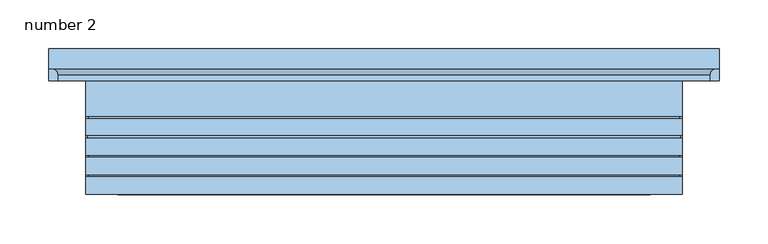
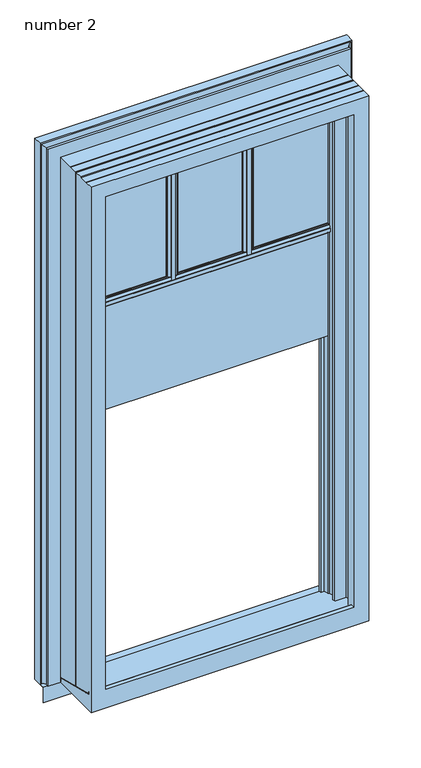
"""IFC4 building model written with IfcOpenShell, lengths in millimetres: window geometry, Window-Exterior-Sierra-Double_Hung-Operating_Unit-18inch_48inch-Width-(Hi-Divide) : number 2."""

from ifc_helpers import new_model, si_unit, point, frame, frame_2d, origin, place, context, project, spatial, polyline, circle_curve, ellipse_curve, trimmed, segment, composite_curve, outline, extrude, source, transform, mapped, element, save
from ifc_brep_helpers import plane_surface, cylinder_surface, revolved_surface, advanced_brep


def number_2_2d71ef64(model_context):
    return source(origin(), model_context, "Body", "SolidModel", [
        extrude(outline(composite_curve([segment(polyline([(-94.1939779, 37.8983982), (-94.1939779, 40.5653982), (-92.6191779, 40.5653982)]), True, "CONTINUOUS"), segment(trimmed(circle_curve(frame_2d((-87.3857184, 38.4281587)), 5.6530426), [point((-92.6191779, 40.5653982))], [point((-87.0396445, 44.0705982))], False, "CARTESIAN"), True, "CONTINUOUS"), segment(polyline([(-87.0396445, 44.0705982), (-87.0396445, 46.6296482), (-79.1233112, 46.6296482), (-79.1233112, 44.0705982)]), True, "CONTINUOUS"), segment(trimmed(circle_curve(frame_2d((-78.7772374, 38.4281587)), 5.6530426), [point((-79.1233112, 44.0705982))], [point((-73.5437779, 40.5653982))], False, "CARTESIAN"), True, "CONTINUOUS"), segment(polyline([(-73.5437779, 40.5653982), (-71.9689779, 40.5653982), (-71.9689779, 37.8983982), (-94.1939779, 37.8983982)]), True, "CONTINUOUS")], self_intersect=False)), frame((0.0, 0.0, 1795.5188733), z_axis=(0.0, 0.0, 1.0), x_axis=(1.0, 0.0, 0.0)), (0.0, 0.0, 1.0), 304.8),
        extrude(outline(composite_curve([segment(polyline([(-94.1939779, 18.8483982), (-71.9689779, 18.8483982), (-71.9689779, 16.1813982), (-73.5437779, 16.1813982)]), True, "CONTINUOUS"), segment(trimmed(circle_curve(frame_2d((-78.7772374, 18.3186378)), 5.6530426), [point((-73.5437779, 16.1813982))], [point((-79.1233112, 12.6761982))], False, "CARTESIAN"), True, "CONTINUOUS"), segment(polyline([(-79.1233112, 12.6761982), (-79.1233112, 10.1171482), (-87.0396445, 10.1171482), (-87.0396445, 12.6761982)]), True, "CONTINUOUS"), segment(trimmed(circle_curve(frame_2d((-87.3857184, 18.3186378)), 5.6530426), [point((-87.0396445, 12.6761982))], [point((-92.6191779, 16.1813982))], False, "CARTESIAN"), True, "CONTINUOUS"), segment(polyline([(-92.6191779, 16.1813982), (-94.1939779, 16.1813982), (-94.1939779, 18.8483982)]), True, "CONTINUOUS")], self_intersect=False)), frame((0.0, 0.0, 1795.5188733), z_axis=(0.0, 0.0, 1.0), x_axis=(1.0, 0.0, 0.0)), (0.0, 0.0, 1.0), 304.8),
        extrude(outline(composite_curve([segment(polyline([(-83.0927539, 18.8483982), (-71.9689779, 18.8483982), (-71.9689779, 14.5562974), (-73.5437779, 14.5562974)]), True, "CONTINUOUS"), segment(trimmed(circle_curve(frame_2d((-78.7772374, 18.3186378)), 6.445487), [point((-73.5437779, 14.5562974))], [point((-79.1233112, 11.8824482))], False, "CARTESIAN"), True, "CONTINUOUS"), segment(polyline([(-79.1233112, 11.8824482), (-79.1233112, 10.1171482), (-87.0396445, 10.1171482), (-87.0396445, 12.6761982)]), True, "CONTINUOUS"), segment(trimmed(circle_curve(frame_2d((-87.3857184, 18.3186378)), 5.6530426), [point((-87.0396445, 12.6761982))], [point((-92.6191779, 16.1813982))], False, "CARTESIAN"), True, "CONTINUOUS"), segment(polyline([(-92.6191779, 16.1813982), (-94.1939779, 16.1813982), (-94.1939779, 18.8483982), (-83.0927539, 18.8483982)]), True, "CONTINUOUS")], self_intersect=False)), frame((0.0, 0.0, 1795.5188733), z_axis=(0.0, 0.0, 1.0), x_axis=(1.0, 0.0, 0.0)), (0.0, 0.0, 1.0), 304.8),
        extrude(outline(composite_curve([segment(polyline([(71.9689779, 37.8983982), (71.9689779, 40.5653982), (73.5437779, 40.5653982)]), True, "CONTINUOUS"), segment(trimmed(circle_curve(frame_2d((78.7772374, 38.4281587)), 5.6530426), [point((73.5437779, 40.5653982))], [point((79.1233112, 44.0705982))], False, "CARTESIAN"), True, "CONTINUOUS"), segment(polyline([(79.1233112, 44.0705982), (79.1233112, 46.6296482), (87.0396445, 46.6296482), (87.0396445, 44.0705982)]), True, "CONTINUOUS"), segment(trimmed(circle_curve(frame_2d((87.3857184, 38.4281587)), 5.6530426), [point((87.0396445, 44.0705982))], [point((92.6191779, 40.5653982))], False, "CARTESIAN"), True, "CONTINUOUS"), segment(polyline([(92.6191779, 40.5653982), (94.1939779, 40.5653982), (94.1939779, 37.8983982), (71.9689779, 37.8983982)]), True, "CONTINUOUS")], self_intersect=False)), frame((0.0, 0.0, 1795.5188733), z_axis=(0.0, 0.0, 1.0), x_axis=(1.0, 0.0, 0.0)), (0.0, 0.0, 1.0), 304.8),
        extrude(outline(composite_curve([segment(polyline([(71.9689779, 18.8483982), (94.1939779, 18.8483982), (94.1939779, 16.1813982), (92.6191779, 16.1813982)]), True, "CONTINUOUS"), segment(trimmed(circle_curve(frame_2d((87.3857184, 18.3186378)), 5.6530426), [point((92.6191779, 16.1813982))], [point((87.0396445, 12.6761982))], False, "CARTESIAN"), True, "CONTINUOUS"), segment(polyline([(87.0396445, 12.6761982), (87.0396445, 10.1171482), (79.1233112, 10.1171482), (79.1233112, 12.6761982)]), True, "CONTINUOUS"), segment(trimmed(circle_curve(frame_2d((78.7772374, 18.3186378)), 5.6530426), [point((79.1233112, 12.6761982))], [point((73.5437779, 16.1813982))], False, "CARTESIAN"), True, "CONTINUOUS"), segment(polyline([(73.5437779, 16.1813982), (71.9689779, 16.1813982), (71.9689779, 18.8483982)]), True, "CONTINUOUS")], self_intersect=False)), frame((0.0, 0.0, 1795.5188733), z_axis=(0.0, 0.0, 1.0), x_axis=(1.0, 0.0, 0.0)), (0.0, 0.0, 1.0), 304.8),
        extrude(outline(composite_curve([segment(polyline([(83.0702018, 18.8483982), (94.1939779, 18.8483982), (94.1939779, 14.5562974), (92.6191779, 14.5562974)]), True, "CONTINUOUS"), segment(trimmed(circle_curve(frame_2d((87.3857184, 18.3186378)), 6.445487), [point((92.6191779, 14.5562974))], [point((87.0396445, 11.8824482))], False, "CARTESIAN"), True, "CONTINUOUS"), segment(polyline([(87.0396445, 11.8824482), (87.0396445, 10.1171482), (79.1233112, 10.1171482), (79.1233112, 12.6761982)]), True, "CONTINUOUS"), segment(trimmed(circle_curve(frame_2d((78.7772374, 18.3186378)), 5.6530426), [point((79.1233112, 12.6761982))], [point((73.5437779, 16.1813982))], False, "CARTESIAN"), True, "CONTINUOUS"), segment(polyline([(73.5437779, 16.1813982), (71.9689779, 16.1813982), (71.9689779, 18.8483982), (83.0702018, 18.8483982)]), True, "CONTINUOUS")], self_intersect=False)), frame((0.0, 0.0, 1795.5188733), z_axis=(0.0, 0.0, 1.0), x_axis=(1.0, 0.0, 0.0)), (0.0, 0.0, 1.0), 304.8),
        extrude(outline(composite_curve([segment(polyline([(37.8983982, 1784.4063733), (37.8983982, 1806.6313733), (40.5653982, 1806.6313733), (40.5653982, 1805.0565733)]), True, "CONTINUOUS"), segment(trimmed(circle_curve(frame_2d((38.4281587, 1799.8231138)), 5.6530426), [point((40.5653982, 1805.0565733))], [point((44.0705982, 1799.47704))], False, "CARTESIAN"), True, "CONTINUOUS"), segment(polyline([(44.0705982, 1799.47704), (48.2171482, 1799.47704), (48.2171482, 1791.5607067), (44.0705982, 1791.5607067)]), True, "CONTINUOUS"), segment(trimmed(circle_curve(frame_2d((38.4281587, 1791.2146328)), 5.6530426), [point((44.0705982, 1791.5607067))], [point((40.5653982, 1785.9811733))], False, "CARTESIAN"), True, "CONTINUOUS"), segment(polyline([(40.5653982, 1785.9811733), (40.5653982, 1784.4063733), (37.8983982, 1784.4063733)]), True, "CONTINUOUS")], self_intersect=False)), frame((-260.35, 0.0, 0.0), z_axis=(1.0, 0.0, 0.0), x_axis=(0.0, 1.0, 0.0)), (0.0, 0.0, 1.0), 520.7),
        extrude(outline(composite_curve([segment(polyline([(18.8483982, 1784.4063733), (16.1813982, 1784.4063733), (16.1813982, 1785.9811733)]), True, "CONTINUOUS"), segment(trimmed(circle_curve(frame_2d((18.3186378, 1791.2146328)), 5.6530426), [point((16.1813982, 1785.9811733))], [point((12.6761982, 1791.5607067))], False, "CARTESIAN"), True, "CONTINUOUS"), segment(polyline([(12.6761982, 1791.5607067), (8.5296482, 1791.5607067), (8.5296482, 1799.47704), (12.6761982, 1799.47704)]), True, "CONTINUOUS"), segment(trimmed(circle_curve(frame_2d((18.3186378, 1799.8231138)), 5.6530426), [point((12.6761982, 1799.47704))], [point((16.1813982, 1805.0565733))], False, "CARTESIAN"), True, "CONTINUOUS"), segment(polyline([(16.1813982, 1805.0565733), (16.1813982, 1806.6313733), (18.8483982, 1806.6313733), (18.8483982, 1784.4063733)]), True, "CONTINUOUS")], self_intersect=False)), frame((-260.35, 0.0, 0.0), z_axis=(1.0, 0.0, 0.0), x_axis=(0.0, 1.0, 0.0)), (0.0, 0.0, 1.0), 520.7),
        extrude(outline(composite_curve([segment(polyline([(18.8483982, 1795.5075973), (18.8483982, 1784.4063733), (16.1813982, 1784.4063733), (16.1813982, 1785.9811733)]), True, "CONTINUOUS"), segment(trimmed(circle_curve(frame_2d((18.3186378, 1791.2146328)), 5.6530426), [point((16.1813982, 1785.9811733))], [point((12.6761982, 1791.5607067))], False, "CARTESIAN"), True, "CONTINUOUS"), segment(polyline([(12.6761982, 1791.5607067), (8.5296482, 1791.5607067), (8.5296482, 1799.47704), (10.2949482, 1799.47704)]), True, "CONTINUOUS"), segment(trimmed(circle_curve(frame_2d((18.3186378, 1799.8231138)), 8.0311494), [point((10.2949482, 1799.47704))], [point((12.2268184, 1805.0565733))], False, "CARTESIAN"), True, "CONTINUOUS"), segment(polyline([(12.2268184, 1805.0565733), (12.2268184, 1806.6313733), (18.8483982, 1806.6313733), (18.8483982, 1795.5075973)]), True, "CONTINUOUS")], self_intersect=False)), frame((-260.35, 0.0, 0.0), z_axis=(1.0, 0.0, 0.0), x_axis=(0.0, 1.0, 0.0)), (0.0, 0.0, 1.0), 520.7),
        extrude(outline(polyline([(-50.9012589, 957.3267373), (-50.1075089, 957.3267373), (-50.1075089, 951.7554125), (57.1246, 925.4832931), (57.1246, 915.4826721), (56.33085, 915.4826721), (56.33085, 924.860538), (-50.9012589, 951.1326574), (-50.9012589, 957.3267373)])), frame((-304.8, 0.0, 0.0), z_axis=(1.0, 0.0, 0.0), x_axis=(0.0, 1.0, 0.0)), (0.0, 0.0, 1.0), 609.6),
        advanced_brep(
        [(289.7632068, 84.19465, 914.4), (289.7632068, 57.575524, 914.4), (289.7632068, 57.575524, 2118.5632068), (289.7632068, 84.19465, 2118.5632068), (322.8412379, 84.82965, 914.4), (321.5640068, 84.19465, 914.4), (321.5640068, 84.19465, 2150.3640068), (322.8412379, 84.82965, 2151.6412379), (325.755083, 86.4286832, 914.4), (325.755083, 86.4286832, 2154.555083), (331.3430068, 87.2508758, 914.4), (331.3430068, 87.2508758, 2160.1430068), (331.3430068, 88.79205, 914.4), (331.3430068, 88.79205, 2160.1430068), (342.3412068, 68.59905, 914.4), (342.3412068, 88.79205, 914.4), (342.3412068, 88.79205, 2171.1412068), (342.3412068, 68.59905, 2171.1412068), (332.9940068, 62.24905, 914.4), (339.3440068, 68.59905, 914.4), (339.3440068, 68.59905, 2168.1440068), (332.9940068, 62.24905, 2161.7940068), (332.9940068, 56.35625, 914.4), (332.9940068, 56.35625, 2161.7940068), (301.625, 19.8870822, 2130.425), (301.625, 17.6010822, 2130.425), (301.625, 17.6010822, 934.3494224), (301.625, 19.8870822, 933.789347), (302.7172, 0.5016996, 2131.5172), (302.7172, -2.6733004, 2131.5172), (302.7172, -2.6733004, 939.3166939), (302.7172, 0.5016996, 938.5388114), (301.625, -19.7004, 2130.425), (301.625, -21.9864039, 2130.425), (301.625, -21.9864039, 944.0484498), (301.625, -19.7004, 943.4883735), (301.625, -39.4941531, 2130.425), (301.625, -41.780157, 2130.425), (301.625, -41.780157, 948.897966), (301.625, -39.4941531, 948.3378896), (-289.7632068, 57.575524, 2118.5632068), (-289.7632068, 84.19465, 2118.5632068), (-321.5640068, 84.19465, 2150.3640068), (-322.8412379, 84.82965, 2151.6412379), (-325.755083, 86.4286832, 2154.555083), (-331.3430068, 87.2508758, 2160.1430068), (-331.3430068, 88.79205, 2160.1430068), (-342.3412068, 88.79205, 2171.1412068), (-342.3412068, 68.59905, 2171.1412068), (-339.3440068, 68.59905, 2168.1440068), (-332.9940068, 62.24905, 2161.7940068), (-332.9940068, 56.35625, 2161.7940068), (304.8, 56.35625, 2133.6), (-304.8, 56.35625, 2133.6), (-304.8, 19.8870822, 2133.6), (304.8, 19.8870822, 2133.6), (-301.625, 19.8870822, 2130.425), (-301.625, 17.6010822, 2130.425), (304.8, 17.6010822, 2133.6), (-304.8, 17.6010822, 2133.6), (-304.8, 0.5016996, 2133.6), (304.8, 0.5016996, 2133.6), (-302.7172, 0.5016996, 2131.5172), (-302.7172, -2.6733004, 2131.5172), (304.8, -2.6733004, 2133.6), (-304.8, -2.6733004, 2133.6), (-304.8, -19.7004, 2133.6), (304.8, -19.7004, 2133.6), (-301.625, -19.7004, 2130.425), (-301.625, -21.9864039, 2130.425), (304.8, -21.9864039, 2133.6), (-304.8, -21.9864039, 2133.6), (-304.8, -39.4941531, 2133.6), (304.8, -39.4941531, 2133.6), (-301.625, -39.4941531, 2130.425), (-301.625, -41.780157, 2130.425), (-304.8, -59.8487004, 2133.6), (304.8, -59.8487004, 2133.6), (304.8, -41.780157, 2133.6), (-304.8, -41.780157, 2133.6), (-289.7632068, 84.19465, 914.4), (-289.7632068, 57.575524, 914.4), (-321.5640068, 84.19465, 914.4), (-322.8412379, 84.82965, 914.4), (-325.755083, 86.4286832, 914.4), (-331.3430068, 87.2508758, 914.4), (-331.3430068, 88.79205, 914.4), (-342.3412068, 88.79205, 914.4), (-342.3412068, 68.59905, 914.4), (-339.3440068, 68.59905, 914.4), (-332.9940068, 62.24905, 914.4), (-332.9940068, 56.35625, 914.4), (-301.625, 19.8870822, 933.789347), (-301.625, 17.6010822, 934.3494224), (-302.7172, 0.5016996, 938.5388114), (-302.7172, -2.6733004, 939.3166939), (-301.625, -19.7004, 943.4883735), (-301.625, -21.9864039, 944.0484498), (-301.625, -39.4941531, 948.3378896), (-301.625, -41.780157, 948.897966), (-304.8, -41.780157, 948.897966), (-304.8, -39.4941531, 948.3378896), (-304.8, -21.9864039, 944.0484498), (-304.8, -19.7004, 943.4883735), (-304.8, -2.6733004, 939.3166939), (-304.8, 0.5016996, 938.5388114), (-304.8, 17.6010822, 934.3494224), (-304.8, 19.8870822, 933.789347), (-304.8, 56.35625, 914.4), (-304.8, -59.8487004, 914.4), (304.8, 19.8870822, 933.789347), (304.8, 17.6010822, 934.3494224), (304.8, 0.5016996, 938.5388114), (304.8, -2.6733004, 939.3166939), (304.8, -19.7004, 943.4883735), (304.8, -21.9864039, 944.0484498), (304.8, -39.4941531, 948.3378896), (304.8, -41.780157, 948.897966), (304.8, -59.8487004, 914.4), (304.8, 56.33085, 914.4), (272.1547286, -59.8487004, 957.3267373), (-272.1547286, -59.8487004, 957.3267373), (-272.1547286, -59.8487004, 2100.9547286), (272.1547286, -59.8487004, 2100.9547286), (264.1437372, 56.33085, 914.4), (-264.1437372, 56.33085, 914.4), (-264.1437372, 56.33085, 924.860538), (264.1437372, 56.33085, 924.860538), (-264.3632068, 57.575524, 914.4), (264.3632068, 57.575524, 914.4), (272.1547286, -50.9012589, 957.3267373), (-272.1547286, -50.9012589, 957.3267373), (272.1547286, -50.9012589, 951.1326574), (-272.1547286, -50.9012589, 951.1326574), (-263.1589309, 50.745736, 926.2289041), (-271.3419286, 50.745736, 926.2289041), (-271.3419286, 35.630345, 929.9322105), (-273.6551976, 35.630345, 929.9322105), (-273.6551976, 4.7593357, 937.4956806), (-262.9778098, 4.7593357, 937.4956806), (-262.9778098, -4.0321944, 939.6496262), (-287.8836, -4.0321944, 939.6496262), (-287.8836, -38.4365384, 948.0787715), (-272.1547286, -38.4365384, 948.0787715), (272.1547286, -38.4365384, 948.0787715), (287.8836, -38.4365384, 948.0787715), (287.8836, -4.0321944, 939.6496262), (262.9778098, -4.0321944, 939.6496262), (262.9778098, 4.7593357, 937.4956806), (273.6551976, 4.7593357, 937.4956806), (273.6551976, 35.630345, 929.9322105), (271.3419286, 35.630345, 929.9322105), (271.3419286, 50.745736, 926.2289041), (263.1589309, 50.745736, 926.2289041), (272.1547286, -38.4365384, 2100.9547286), (-272.1547286, -38.4365384, 2100.9547286), (-287.8836, -38.4365384, 2116.6836), (287.8836, -38.4365384, 2116.6836), (287.8836, -4.0321944, 2116.6836), (-287.8836, -4.0321944, 2116.6836), (-262.9778098, -4.0321944, 2091.7778098), (262.9778098, -4.0321944, 2091.7778098), (262.9778098, 4.7593357, 2091.7778098), (-262.9778098, 4.7593357, 2091.7778098), (-273.6551976, 4.7593357, 2102.4551976), (273.6551976, 4.7593357, 2102.4551976), (273.6551976, 35.630345, 2102.4551976), (-273.6551976, 35.630345, 2102.4551976), (-271.3419286, 35.630345, 2100.1419286), (271.3419286, 35.630345, 2100.1419286), (271.3419286, 50.745736, 2100.1419286), (-271.3419286, 50.745736, 2100.1419286), (-263.1589309, 50.745736, 2091.9589309), (263.1589309, 50.745736, 2091.9589309), (264.3632068, 57.575524, 2093.1632068), (-264.3632068, 57.575524, 2093.1632068)],
        [
            (0, 1),
            (1, 2),
            (2, 3),
            (3, 0),
            (4, 5),
            (5, 6),
            (6, 7),
            (7, 4),
            (8, 4, circle_curve(frame((322.8412379, 88.28405, 914.4), z_axis=(0.0, 0.0, -1.0), x_axis=(0.0, -1.0, 0.0)), 3.4544)),
            (7, 9, ellipse_curve(frame((322.8412379, 88.28405, 2151.6412379), z_axis=(-0.7071067811865475, 0.0, 0.7071067811865475), x_axis=(0.7071067811865474, 0.0, 0.7071067811865476)), 4.8852593, 3.4544)),
            (9, 8),
            (10, 8, circle_curve(frame((328.9046068, 84.42325, 914.4), z_axis=(0.0, 0.0, 1.0), x_axis=(0.0, -1.0, 0.0)), 3.7338)),
            (9, 11, ellipse_curve(frame((328.9046068, 84.42325, 2157.7046068), z_axis=(0.7071067811865475, 0.0, -0.7071067811865475), x_axis=(-0.7071067811865474, 0.0, -0.7071067811865476)), 5.2803906, 3.7338)),
            (11, 10),
            (12, 10),
            (11, 13),
            (13, 12),
            (14, 15),
            (15, 16),
            (16, 17),
            (17, 14),
            (18, 19, circle_curve(frame((339.3440068, 62.24905, 914.4), z_axis=(0.0, 0.0, -1.0), x_axis=(0.0, -1.0, 0.0)), 6.35)),
            (19, 20),
            (20, 21, ellipse_curve(frame((339.3440068, 62.24905, 2168.1440068), z_axis=(-0.7071067811865475, 0.0, 0.7071067811865475), x_axis=(0.7071067811865474, 0.0, 0.7071067811865476)), 8.9802561, 6.35)),
            (21, 18),
            (22, 18),
            (21, 23),
            (23, 22),
            (24, 25),
            (25, 26),
            (26, 27),
            (27, 24),
            (28, 29),
            (29, 30),
            (30, 31),
            (31, 28),
            (32, 33),
            (33, 34),
            (34, 35),
            (35, 32),
            (36, 37),
            (37, 38),
            (38, 39),
            (39, 36),
            (2, 40),
            (40, 41),
            (41, 3),
            (6, 42),
            (42, 43),
            (43, 7),
            (43, 44, ellipse_curve(frame((-322.8412379, 88.28405, 2151.6412379), z_axis=(-0.7071067811865475, 0.0, -0.7071067811865475), x_axis=(-0.7071067811865476, 0.0, 0.7071067811865474)), 4.8852593, 3.4544)),
            (44, 9),
            (44, 45, ellipse_curve(frame((-328.9046068, 84.42325, 2157.7046068), z_axis=(0.7071067811865475, 0.0, 0.7071067811865475), x_axis=(0.7071067811865476, 0.0, -0.7071067811865474)), 5.2803906, 3.7338)),
            (45, 11),
            (45, 46),
            (46, 13),
            (16, 47),
            (47, 48),
            (48, 17),
            (20, 49),
            (49, 50, ellipse_curve(frame((-339.3440068, 62.24905, 2168.1440068), z_axis=(-0.7071067811865475, 0.0, -0.7071067811865475), x_axis=(-0.7071067811865476, 0.0, 0.7071067811865474)), 8.9802561, 6.35)),
            (50, 21),
            (50, 51),
            (51, 23),
            (52, 53),
            (53, 54),
            (54, 55),
            (55, 52),
            (24, 56),
            (56, 57),
            (57, 25),
            (58, 59),
            (59, 60),
            (60, 61),
            (61, 58),
            (28, 62),
            (62, 63),
            (63, 29),
            (64, 65),
            (65, 66),
            (66, 67),
            (67, 64),
            (32, 68),
            (68, 69),
            (69, 33),
            (70, 71),
            (71, 72),
            (72, 73),
            (73, 70),
            (36, 74),
            (74, 75),
            (75, 37),
            (76, 77),
            (77, 78),
            (78, 79),
            (79, 76),
            (80, 41),
            (40, 81),
            (81, 80),
            (42, 82),
            (82, 83),
            (83, 43),
            (83, 84, circle_curve(frame((-322.8412379, 88.28405, 914.4), z_axis=(0.0, 0.0, -1.0), x_axis=(0.0, -1.0, 0.0)), 3.4544)),
            (84, 44),
            (84, 85, circle_curve(frame((-328.9046068, 84.42325, 914.4), z_axis=(0.0, 0.0, 1.0), x_axis=(0.0, -1.0, 0.0)), 3.7338)),
            (85, 45),
            (86, 46),
            (85, 86),
            (47, 87),
            (87, 88),
            (88, 48),
            (49, 89),
            (89, 90, circle_curve(frame((-339.3440068, 62.24905, 914.4), z_axis=(0.0, 0.0, -1.0), x_axis=(0.0, -1.0, 0.0)), 6.35)),
            (90, 50),
            (91, 51),
            (90, 91),
            (56, 92),
            (92, 93),
            (93, 57),
            (62, 94),
            (94, 95),
            (95, 63),
            (68, 96),
            (96, 97),
            (97, 69),
            (74, 98),
            (98, 99),
            (99, 75),
            (79, 100),
            (100, 101),
            (101, 72),
            (71, 102),
            (102, 103),
            (103, 66),
            (65, 104),
            (104, 105),
            (105, 60),
            (59, 106),
            (106, 107),
            (107, 54),
            (53, 108),
            (108, 109),
            (109, 76),
            (55, 110),
            (110, 111),
            (111, 58),
            (61, 112),
            (112, 113),
            (113, 64),
            (67, 114),
            (114, 115),
            (115, 70),
            (73, 116),
            (116, 117),
            (117, 78),
            (77, 118),
            (118, 119),
            (119, 52),
            (109, 118),
            (120, 121),
            (121, 122),
            (122, 123),
            (123, 120),
            (124, 125),
            (125, 126),
            (126, 127),
            (127, 124),
            (5, 0),
            (80, 82),
            (15, 12),
            (86, 87),
            (19, 14),
            (88, 89),
            (119, 22),
            (91, 108),
            (107, 92),
            (27, 110),
            (93, 106),
            (111, 26),
            (105, 94),
            (31, 112),
            (95, 104),
            (113, 30),
            (103, 96),
            (35, 114),
            (97, 102),
            (115, 34),
            (101, 98),
            (39, 116),
            (99, 100),
            (117, 38),
            (81, 128),
            (128, 125),
            (124, 129),
            (129, 1),
            (120, 130),
            (130, 131),
            (131, 121),
            (130, 132),
            (132, 133),
            (133, 131),
            (126, 134),
            (134, 135),
            (135, 136),
            (136, 137),
            (137, 138),
            (138, 139),
            (139, 140),
            (140, 141),
            (141, 142),
            (142, 143),
            (143, 133),
            (132, 144),
            (144, 145),
            (145, 146),
            (146, 147),
            (147, 148),
            (148, 149),
            (149, 150),
            (150, 151),
            (151, 152),
            (152, 153),
            (153, 127),
            (123, 154),
            (154, 144),
            (154, 155),
            (155, 143),
            (142, 156),
            (156, 157),
            (157, 145),
            (157, 158),
            (158, 146),
            (158, 159),
            (159, 141),
            (140, 160),
            (160, 161),
            (161, 147),
            (161, 162),
            (162, 148),
            (162, 163),
            (163, 139),
            (138, 164),
            (164, 165),
            (165, 149),
            (165, 166),
            (166, 150),
            (166, 167),
            (167, 137),
            (136, 168),
            (168, 169),
            (169, 151),
            (169, 170),
            (170, 152),
            (170, 171),
            (171, 135),
            (134, 172),
            (172, 173),
            (173, 153),
            (173, 174),
            (174, 129),
            (174, 175),
            (175, 128),
            (122, 155),
            (156, 159),
            (160, 163),
            (164, 167),
            (168, 171),
            (172, 175),
        ],
        [
            plane_surface(frame((289.7632068, 57.575524, 914.4), z_axis=(-1.0, 0.0, 0.0), x_axis=(0.0, 0.0, 1.0))),
            plane_surface(frame((321.5640068, 84.19465, 914.4), z_axis=(-0.44518462388465885, 0.8954388034124247, 0.0), x_axis=(0.0, 0.0, 1.0))),
            revolved_surface(polyline([(322.8412379, 84.82964999999999, 2155.095637878884), (322.8412379, 84.82964999999999, 914.4)]), (322.8412379, 88.28405, 914.4), (0.0, 0.0, 1.0)),
            cylinder_surface(frame((328.9046068, 84.42325, 914.4), z_axis=(0.0, 0.0, -1.0), x_axis=(0.0, -1.0, 0.0)), 3.7338),
            plane_surface(frame((331.3430068, 87.2508758, 914.4), z_axis=(-1.0, 0.0, 0.0), x_axis=(0.0, 0.0, 1.0))),
            plane_surface(frame((342.3412068, 88.79205, 914.4), z_axis=(1.0, 0.0, 0.0), x_axis=(0.0, 0.0, 1.0))),
            revolved_surface(polyline([(339.3440068, 55.899049999999995, 2174.494006785102), (339.3440068, 55.899049999999995, 914.4)]), (339.3440068, 62.24905, 914.4), (0.0, 0.0, 1.0)),
            plane_surface(frame((332.9940068, 62.24905, 914.4), z_axis=(1.0, 0.0, 0.0), x_axis=(0.0, 0.0, 1.0))),
            plane_surface(frame((301.625, 19.8870822, 914.4), z_axis=(1.0, 0.0, 0.0), x_axis=(0.0, 0.0, 1.0))),
            plane_surface(frame((302.7172, 0.5016996, 914.4), z_axis=(1.0, 0.0, 0.0), x_axis=(0.0, 0.0, 1.0))),
            plane_surface(frame((301.625, -19.7004, 914.4), z_axis=(1.0, 0.0, 0.0), x_axis=(0.0, 0.0, 1.0))),
            plane_surface(frame((301.625, -39.4941531, 914.4), z_axis=(1.0, 0.0, 0.0), x_axis=(0.0, 0.0, 1.0))),
            plane_surface(frame((289.7632068, 57.575524, 2118.5632068), z_axis=(0.0, 0.0, -1.0), x_axis=(-1.0, 0.0, 0.0))),
            plane_surface(frame((321.5640068, 84.19465, 2150.3640068), z_axis=(0.0, 0.8954388034124309, -0.4451846238846465), x_axis=(-1.0, 0.0, 0.0))),
            revolved_surface(polyline([(-326.29563787888475, 84.82964999999999, 2151.6412379), (326.29563787888463, 84.82964999999999, 2151.6412379)]), (304.8, 88.28405, 2151.6412379), (-1.0, 0.0, 0.0)),
            cylinder_surface(frame((304.8, 84.42325, 2157.7046068), z_axis=(1.0, 0.0, 0.0), x_axis=(0.0, -1.0, 0.0)), 3.7338),
            plane_surface(frame((331.3430068, 87.2508758, 2160.1430068), z_axis=(0.0, 0.0, -1.0), x_axis=(-1.0, 0.0, 0.0))),
            plane_surface(frame((342.3412068, 88.79205, 2171.1412068), z_axis=(0.0, 0.0, 1.0), x_axis=(-1.0, 0.0, 0.0))),
            revolved_surface(polyline([(-345.69400678510175, 55.899049999999995, 2168.1440068), (345.69400678510186, 55.899049999999995, 2168.1440068)]), (304.8, 62.24905, 2168.1440068), (-1.0, 0.0, 0.0)),
            plane_surface(frame((332.9940068, 62.24905, 2161.7940068), z_axis=(0.0, 0.0, 1.0), x_axis=(-1.0, 0.0, 0.0))),
            plane_surface(frame((304.8, 56.35625, 2133.6), z_axis=(0.0, 0.0, 1.0), x_axis=(-1.0, 0.0, 0.0))),
            plane_surface(frame((301.625, 19.8870822, 2130.425), z_axis=(0.0, 0.0, 1.0), x_axis=(-1.0, 0.0, 0.0))),
            plane_surface(frame((304.8, 17.6010822, 2133.6), z_axis=(0.0, 0.0, 1.0), x_axis=(-1.0, 0.0, 0.0))),
            plane_surface(frame((302.7172, 0.5016996, 2131.5172), z_axis=(0.0, 0.0, 1.0), x_axis=(-1.0, 0.0, 0.0))),
            plane_surface(frame((304.8, -2.6733004, 2133.6), z_axis=(0.0, 0.0, 1.0), x_axis=(-1.0, 0.0, 0.0))),
            plane_surface(frame((301.625, -19.7004, 2130.425), z_axis=(0.0, 0.0, 1.0), x_axis=(-1.0, 0.0, 0.0))),
            plane_surface(frame((304.8, -21.9864039, 2133.6), z_axis=(0.0, 0.0, 1.0), x_axis=(-1.0, 0.0, 0.0))),
            plane_surface(frame((301.625, -39.4941531, 2130.425), z_axis=(0.0, 0.0, 1.0), x_axis=(-1.0, 0.0, 0.0))),
            plane_surface(frame((304.8, -41.780157, 2133.6), z_axis=(0.0, 0.0, 1.0), x_axis=(-1.0, 0.0, 0.0))),
            plane_surface(frame((-289.7632068, 57.575524, 2118.5632068), z_axis=(1.0, 0.0, 0.0), x_axis=(0.0, 0.0, -1.0))),
            plane_surface(frame((-321.5640068, 84.19465, 2150.3640068), z_axis=(0.44518462388465885, 0.8954388034124247, 0.0), x_axis=(0.0, 0.0, -1.0))),
            revolved_surface(polyline([(-322.8412379, 84.82964999999999, 914.4000000000001), (-322.8412379, 84.82964999999999, 2155.0956378788846)]), (-322.8412379, 88.28405, 2133.6), (0.0, 0.0, -1.0)),
            cylinder_surface(frame((-328.9046068, 84.42325, 2133.6), z_axis=(0.0, 0.0, 1.0), x_axis=(0.0, -1.0, 0.0)), 3.7338),
            plane_surface(frame((-331.3430068, 87.2508758, 2160.1430068), z_axis=(1.0, 0.0, 0.0), x_axis=(0.0, 0.0, -1.0))),
            plane_surface(frame((-342.3412068, 88.79205, 2171.1412068), z_axis=(-1.0, 0.0, 0.0), x_axis=(0.0, 0.0, -1.0))),
            revolved_surface(polyline([(-339.3440068, 55.899049999999995, 914.4000000000001), (-339.3440068, 55.899049999999995, 2174.494006785102)]), (-339.3440068, 62.24905, 2133.6), (0.0, 0.0, -1.0)),
            plane_surface(frame((-332.9940068, 62.24905, 2161.7940068), z_axis=(-1.0, 0.0, 0.0), x_axis=(0.0, 0.0, -1.0))),
            plane_surface(frame((-301.625, 19.8870822, 2130.425), z_axis=(-1.0, 0.0, 0.0), x_axis=(0.0, 0.0, -1.0))),
            plane_surface(frame((-302.7172, 0.5016996, 2131.5172), z_axis=(-1.0, 0.0, 0.0), x_axis=(0.0, 0.0, -1.0))),
            plane_surface(frame((-301.625, -19.7004, 2130.425), z_axis=(-1.0, 0.0, 0.0), x_axis=(0.0, 0.0, -1.0))),
            plane_surface(frame((-301.625, -39.4941531, 2130.425), z_axis=(-1.0, 0.0, 0.0), x_axis=(0.0, 0.0, -1.0))),
            plane_surface(frame((-304.8, -7.14375, 914.4), z_axis=(-1.0, 0.0, 0.0), x_axis=(0.0, -1.0, 0.0))),
            plane_surface(frame((304.8, -7.14375, 914.4), z_axis=(1.0, 0.0, 0.0), x_axis=(0.0, -1.0, 0.0))),
            plane_surface(frame((-304.8, -59.8487004, 914.4), z_axis=(0.0, -1.0, 0.0), x_axis=(1.0, 0.0, 0.0))),
            plane_surface(frame((-304.8, 56.33085, 924.860538), z_axis=(0.0, 1.0, 0.0), x_axis=(1.0, 0.0, 0.0))),
            plane_surface(frame((289.7632068, 84.19465, 914.4), z_axis=(0.0, 1.0, 0.0), x_axis=(0.0, 0.0, 1.0))),
            plane_surface(frame((331.3430068, 88.79205, 914.4), z_axis=(0.0, 1.0, 0.0), x_axis=(0.0, 0.0, 1.0))),
            plane_surface(frame((342.3412068, 68.59905, 914.4), z_axis=(0.0, -1.0, 0.0), x_axis=(0.0, 0.0, 1.0))),
            plane_surface(frame((332.9940068, 56.35625, 914.4), z_axis=(0.0, -1.0, 0.0), x_axis=(0.0, 0.0, 1.0))),
            plane_surface(frame((304.8, 19.8870822, 914.4), z_axis=(0.0, -1.0, 0.0), x_axis=(0.0, 0.0, 1.0))),
            plane_surface(frame((301.625, 17.6010822, 914.4), z_axis=(0.0, 1.0, 0.0), x_axis=(0.0, 0.0, 1.0))),
            plane_surface(frame((304.8, 0.5016996, 914.4), z_axis=(0.0, -1.0, 0.0), x_axis=(0.0, 0.0, 1.0))),
            plane_surface(frame((302.7172, -2.6733004, 914.4), z_axis=(0.0, 1.0, 0.0), x_axis=(0.0, 0.0, 1.0))),
            plane_surface(frame((304.8, -19.7004, 914.4), z_axis=(0.0, -1.0, 0.0), x_axis=(0.0, 0.0, 1.0))),
            plane_surface(frame((301.625, -21.9864039, 914.4), z_axis=(0.0, 1.0, 0.0), x_axis=(0.0, 0.0, 1.0))),
            plane_surface(frame((304.8, -39.4941531, 914.4), z_axis=(0.0, -1.0, 0.0), x_axis=(0.0, 0.0, 1.0))),
            plane_surface(frame((301.625, -41.780157, 914.4), z_axis=(0.0, 1.0, 0.0), x_axis=(0.0, 0.0, 1.0))),
            plane_surface(frame((-304.8, -34.2215252, 914.4), z_axis=(0.0, 0.0, -1.0), x_axis=(1.0, 0.0, 0.0))),
            plane_surface(frame((-304.8, -59.8487004, 957.3267373), z_axis=(0.0, 0.0, 1.0), x_axis=(1.0, 0.0, 0.0))),
            plane_surface(frame((-304.8, -50.9012589, 957.3267373), z_axis=(0.0, 1.0, 0.0), x_axis=(1.0, 0.0, 0.0))),
            plane_surface(frame((-304.8, -50.9012589, 951.1326574), z_axis=(0.0, 0.23796439002605316, 0.9712738795414652), x_axis=(1.0, 0.0, 0.0))),
            plane_surface(frame((272.1547286, -59.8487004, 914.4), z_axis=(-1.0, 0.0, 0.0), x_axis=(0.0, 0.0, 1.0))),
            plane_surface(frame((272.1547286, -38.4365384, 914.4), z_axis=(0.0, 1.0, 0.0), x_axis=(0.0, 0.0, 1.0))),
            plane_surface(frame((287.8836, -38.4365384, 914.4), z_axis=(-1.0, 0.0, 0.0), x_axis=(0.0, 0.0, 1.0))),
            plane_surface(frame((287.8836, -4.0321944, 914.4), z_axis=(0.0, -1.0, 0.0), x_axis=(0.0, 0.0, 1.0))),
            plane_surface(frame((262.9778098, -4.0321944, 914.4), z_axis=(-1.0, 0.0, 0.0), x_axis=(0.0, 0.0, 1.0))),
            plane_surface(frame((262.9778098, 4.7593357, 914.4), z_axis=(0.0, 1.0, 0.0), x_axis=(0.0, 0.0, 1.0))),
            plane_surface(frame((273.6551976, 4.7593357, 914.4), z_axis=(-1.0, 0.0, 0.0), x_axis=(0.0, 0.0, 1.0))),
            plane_surface(frame((273.6551976, 35.630345, 914.4), z_axis=(0.0, -1.0, 0.0), x_axis=(0.0, 0.0, 1.0))),
            plane_surface(frame((271.3419286, 35.630345, 914.4), z_axis=(-1.0, 0.0, 0.0), x_axis=(0.0, 0.0, 1.0))),
            plane_surface(frame((271.3419286, 50.745736, 914.4), z_axis=(0.0, -1.0, 0.0), x_axis=(0.0, 0.0, 1.0))),
            plane_surface(frame((263.1589309, 50.745736, 914.4), z_axis=(-0.984807753012208, 0.1736481776669311, 0.0), x_axis=(0.0, 0.0, 1.0))),
            plane_surface(frame((264.3632068, 57.575524, 914.4), z_axis=(0.0, 1.0, 0.0), x_axis=(0.0, 0.0, 1.0))),
            plane_surface(frame((272.1547286, -59.8487004, 2100.9547286), z_axis=(0.0, 0.0, -1.0), x_axis=(-1.0, 0.0, 0.0))),
            plane_surface(frame((287.8836, -38.4365384, 2116.6836), z_axis=(0.0, 0.0, -1.0), x_axis=(-1.0, 0.0, 0.0))),
            plane_surface(frame((262.9778098, -4.0321944, 2091.7778098), z_axis=(0.0, 0.0, -1.0), x_axis=(-1.0, 0.0, 0.0))),
            plane_surface(frame((273.6551976, 4.7593357, 2102.4551976), z_axis=(0.0, 0.0, -1.0), x_axis=(-1.0, 0.0, 0.0))),
            plane_surface(frame((271.3419286, 35.630345, 2100.1419286), z_axis=(0.0, 0.0, -1.0), x_axis=(-1.0, 0.0, 0.0))),
            plane_surface(frame((263.1589309, 50.745736, 2091.9589309), z_axis=(0.0, 0.17364817766694474, -0.9848077530122056), x_axis=(-1.0, 0.0, 0.0))),
            plane_surface(frame((-272.1547286, -59.8487004, 2100.9547286), z_axis=(1.0, 0.0, 0.0), x_axis=(0.0, 0.0, -1.0))),
            plane_surface(frame((-287.8836, -38.4365384, 2116.6836), z_axis=(1.0, 0.0, 0.0), x_axis=(0.0, 0.0, -1.0))),
            plane_surface(frame((-262.9778098, -4.0321944, 2091.7778098), z_axis=(1.0, 0.0, 0.0), x_axis=(0.0, 0.0, -1.0))),
            plane_surface(frame((-273.6551976, 4.7593357, 2102.4551976), z_axis=(1.0, 0.0, 0.0), x_axis=(0.0, 0.0, -1.0))),
            plane_surface(frame((-271.3419286, 35.630345, 2100.1419286), z_axis=(1.0, 0.0, 0.0), x_axis=(0.0, 0.0, -1.0))),
            plane_surface(frame((-263.1589309, 50.745736, 2091.9589309), z_axis=(0.984807753012208, 0.1736481776669311, 0.0), x_axis=(0.0, 0.0, -1.0))),
        ],
        [
            (0, [[1, 2, 3, 4]]),
            (1, [[5, 6, 7, 8]]),
            (2, [[9, -8, 10, 11]]),
            (3, [[12, -11, 13, 14]]),
            (4, [[15, -14, 16, 17]]),
            (5, [[18, 19, 20, 21]]),
            (6, [[22, 23, 24, 25]]),
            (7, [[26, -25, 27, 28]]),
            (8, [[29, 30, 31, 32]]),
            (9, [[33, 34, 35, 36]]),
            (10, [[37, 38, 39, 40]]),
            (11, [[41, 42, 43, 44]]),
            (12, [[-3, 45, 46, 47]]),
            (13, [[48, 49, 50, -7]]),
            (14, [[-10, -50, 51, 52]]),
            (15, [[-13, -52, 53, 54]]),
            (16, [[-16, -54, 55, 56]]),
            (17, [[57, 58, 59, -20]]),
            (18, [[60, 61, 62, -24]]),
            (19, [[-27, -62, 63, 64]]),
            (20, [[65, 66, 67, 68]]),
            (21, [[69, 70, 71, -29]]),
            (22, [[72, 73, 74, 75]]),
            (23, [[76, 77, 78, -33]]),
            (24, [[79, 80, 81, 82]]),
            (25, [[83, 84, 85, -37]]),
            (26, [[86, 87, 88, 89]]),
            (27, [[90, 91, 92, -41]]),
            (28, [[93, 94, 95, 96]]),
            (29, [[97, -46, 98, 99]]),
            (30, [[100, 101, 102, -49]]),
            (31, [[-51, -102, 103, 104]]),
            (32, [[-53, -104, 105, 106]]),
            (33, [[107, -55, -106, 108]]),
            (34, [[109, 110, 111, -58]]),
            (35, [[112, 113, 114, -61]]),
            (36, [[115, -63, -114, 116]]),
            (37, [[-70, 117, 118, 119]]),
            (38, [[-77, 120, 121, 122]]),
            (39, [[-84, 123, 124, 125]]),
            (40, [[-91, 126, 127, 128]]),
            (41, [[-96, 129, 130, 131, -87, 132, 133, 134, -80, 135, 136, 137, -73, 138, 139, 140, -66, 141, 142, 143]]),
            (42, [[-68, 144, 145, 146, -75, 147, 148, 149, -82, 150, 151, 152, -89, 153, 154, 155, -94, 156, 157, 158]]),
            (43, [[-143, 159, -156, -93], [160, 161, 162, 163]]),
            (44, [[164, 165, 166, 167]]),
            (45, [[168, -4, -47, -97, 169, -100, -48, -6]]),
            (46, [[170, -17, -56, -107, 171, -109, -57, -19]]),
            (47, [[172, -21, -59, -111, 173, -112, -60, -23]]),
            (48, [[-158, 174, -28, -64, -115, 175, -141, -65]]),
            (49, [[-67, -140, 176, -117, -69, -32, 177, -144]]),
            (50, [[-71, -119, 178, -138, -72, -146, 179, -30]]),
            (51, [[-74, -137, 180, -120, -76, -36, 181, -147]]),
            (52, [[-78, -122, 182, -135, -79, -149, 183, -34]]),
            (53, [[-81, -134, 184, -123, -83, -40, 185, -150]]),
            (54, [[-85, -125, 186, -132, -86, -152, 187, -38]]),
            (55, [[-88, -131, 188, -126, -90, -44, 189, -153]]),
            (56, [[-92, -128, 190, -129, -95, -155, 191, -42]]),
            (57, [[-142, -175, -116, -113, -173, -110, -171, -108, -105, -103, -101, -169, -99, 192, 193, -164, 194, 195, -1, -168, -5, -9, -12, -15, -170, -18, -172, -22, -26, -174, -157, -159]]),
            (58, [[-160, 196, 197, 198]]),
            (59, [[-197, 199, 200, 201]]),
            (60, [[-130, -190, -127, -188]]),
            (60, [[-133, -186, -124, -184]]),
            (60, [[-136, -182, -121, -180]]),
            (60, [[-139, -178, -118, -176]]),
            (60, [[-145, -177, -31, -179]]),
            (60, [[-148, -181, -35, -183]]),
            (60, [[-151, -185, -39, -187]]),
            (60, [[-154, -189, -43, -191]]),
            (60, [[-166, 202, 203, 204, 205, 206, 207, 208, 209, 210, 211, 212, -200, 213, 214, 215, 216, 217, 218, 219, 220, 221, 222, 223]]),
            (61, [[224, 225, -213, -199, -196, -163]]),
            (62, [[226, 227, -211, 228, 229, 230, -214, -225]]),
            (63, [[231, 232, -215, -230]]),
            (64, [[233, 234, -209, 235, 236, 237, -216, -232]]),
            (65, [[238, 239, -217, -237]]),
            (66, [[240, 241, -207, 242, 243, 244, -218, -239]]),
            (67, [[245, 246, -219, -244]]),
            (68, [[247, 248, -205, 249, 250, 251, -220, -246]]),
            (69, [[252, 253, -221, -251]]),
            (70, [[254, 255, -203, 256, 257, 258, -222, -253]]),
            (71, [[259, 260, -194, -167, -223, -258]]),
            (72, [[-195, -260, 261, 262, -192, -98, -45, -2]]),
            (73, [[-162, 263, -226, -224]]),
            (74, [[-229, 264, -233, -231]]),
            (75, [[-236, 265, -240, -238]]),
            (76, [[-243, 266, -247, -245]]),
            (77, [[-250, 267, -254, -252]]),
            (78, [[-257, 268, -261, -259]]),
            (79, [[-263, -161, -198, -201, -212, -227]]),
            (80, [[-264, -228, -210, -234]]),
            (81, [[-265, -235, -208, -241]]),
            (82, [[-266, -242, -206, -248]]),
            (83, [[-267, -249, -204, -255]]),
            (84, [[-262, -268, -256, -202, -165, -193]]),
        ],
    ),
        extrude(outline(polyline([(56.35625, 879.8504162), (56.35625, 915.510409), (86.4701703, 915.510409), (86.4701703, 914.3989345), (57.7255425, 914.3989345), (57.7255425, 879.8504162), (56.35625, 879.8504162)])), frame((-342.3412068, 0.0, 0.0), z_axis=(1.0, 0.0, 0.0), x_axis=(0.0, 1.0, 0.0)), (0.0, 0.0, 1.0), 684.6824136),
        extrude(outline(polyline([(-260.54685, 37.8983982), (260.54685, 37.8983982), (260.54685, 18.8493162), (-260.54685, 18.8493162), (-260.54685, 37.8983982)])), frame((0.0, 0.0, 1543.84375), z_axis=(0.0, 0.0, 1.0), x_axis=(1.0, 0.0, 0.0)), (0.0, 0.0, 1.0), 545.5031),
    ])


if __name__ == "__main__":
    model = new_model("IFC4")
    model_context = context("Model", 3, world=origin())
    ifc_project = project(units=[si_unit("LENGTHUNIT", "METRE", prefix="MILLI")], contexts=[model_context])
    site = spatial("IfcSite", under=ifc_project)
    building = spatial("IfcBuilding", under=site)
    placement = place(None, origin())
    number_2_shape = number_2_2d71ef64(model_context)
    element("IfcWindow", 1, ObjectType="Window-Exterior-Sierra-Double_Hung-Operating_Unit-18inch_48inch-Width-(Hi-Divide) : number 2", at=placement, inside=building, context=model_context, shape_type="MappedRepresentation", body=[
        mapped(number_2_shape, transform((0.0, 0.0, 0.0), x_axis=(1.0, 0.0, 0.0), y_axis=(0.0, 1.0, 0.0), z_axis=(0.0, 0.0, 1.0))),
    ])
    save(model, "model.ifc")

# Revit data of these elements
# Type "Window-Exterior-Sierra-Double_Hung-Operating_Unit-18inch_48inch-Width-(Hi-Divide) : number 2"
#   Type Mark = "53"
#   URL = "http://www.sierrapacificwindows.com"
#   Simulite Note = "Custom Simulite Options Available"
#   Product data url = "https://bimobject.com/sierrapacificwindows/product/sierrapacificwindows_double-hung-windows"
#   Product Page URL = "http://www.sierrapacificwindows.com/double-hung-windows.cfm"
#   Product Documentation Link = "http://www.sierrapacificwindows.com/architectural/drawings/pdfs/c-dhc_16.1.pdf"
#   Model = "C-DHC-2436"
#   Manufacturer = "Sierra Pacific Windows"
#   Jamb Extension Note = "Extension Jamb may be applied on some applications. Contact your SPW sales rep. for more information"
#   Glass Type = "Insulated Glass"
#   Description = "Energy efficient, durable, and secure window"
#   Construction Type = "Wood/Clad"
#   Assembly Code = "B2030230"
#   Window Pane Thickness = 0' - 0 3/4"
#   Vertical Simulite Length = 1' - 10"
#   Thickness = 0' - 1 3/4"
#   Simulite Wood Thickness Vertical = 0' - 0 11/32"
#   Simulite Wood Thickness Horizontal = 0' - 0 13/32"
#   Simulite Width = 0' - 0 7/8"
#   Simulite Clad Thickness Vertical = 0' - 0 11/32"
#   Simulite Clad Thickness Horizontal = 0' - 0 13/32"
#   Setback = 0' - 0"
#   Rough Width = 2' - 0 3/4"
#   Rough Height = 4' - 0 3/4"
#   Interior Setback = 0' - 0"
#   Horizontal Simulite Length = 1' - 8 1/2"
#   Hi Divide Horizontal Height = 1' - 0"
#   Half Window Height = 2' - 0"
#   Frame Width = 2' - 0"
#   Height = 4' - 0"
#   Width = 2' - 0"
#   Frame Height = 4' - 0"
#   First Simulite Width = 0' - 6.54167"
#   Default Sill Height = 3' - 0"
#   Actual Width = 2' - 0"
#   Actual Height = 4' - 0"
#   Actual Half Width = 1' - 0"
#   Actual Glass Width = 1' - 7 5/8"
#   Actual Glass Height = 1' - 8 1/2"
#   Wood Frame = yes
#   Total Number of Lites Per Panel = 4
#   Simulite Hi Divide Option = yes
#   Number of Vertical Simulites Greater than One = 2
#   Number of Hi Divide Verticals = 2
#   Clad Frame = no
#   Actual Vertical Simulites ( Hi Divide ) = 2
#   Vertical Simulite Type = element 491478
#   Interior Simulite = Wood - Sierra Pacific - Pine
#   Interior Panel Material = Wood - Sierra Pacific - Pine
#   Horizontal Simulite Type = element 491483
#   Glass = Glass - Sierra Doors - Clear
#   Frame = douglas fir
#   Exterior Simulite = Paint - Sierra Pacific - White 001
#   Exterior Panel Material = Paint - Sierra Pacific - White 001
#   Exterior Clad Material = Paint - Sierra Pacific - White 001
#   Wall Closure = (empty or 0)
# Element 1 (IfcWindow, "Window-Exterior-Sierra-Double_Hung-Operating_Unit-18inch_48inch-Width-(Hi-Divide) : number 2")
#   Materials on its faces: "Wood - Sierra Pacific - Pine", "Paint - Sierra Pacific - White 001", "douglas fir", "Glass - Sierra Doors - Clear"
# Materials
#   "Wood - Sierra Pacific - Pine": class "Miscellaneous", colour RGB 136 105 68, transparency 0
#   "Glass - Sierra Doors - Clear": class "Glass", colour RGB 0 0 255, transparency 0.75
#   "douglas fir": class "Generic", colour RGB 120 120 120, transparency 0, Cost = 0
#   "Paint - Sierra Pacific - White 001": class "Miscellaneous", colour RGB 111 112 111, transparency 0
